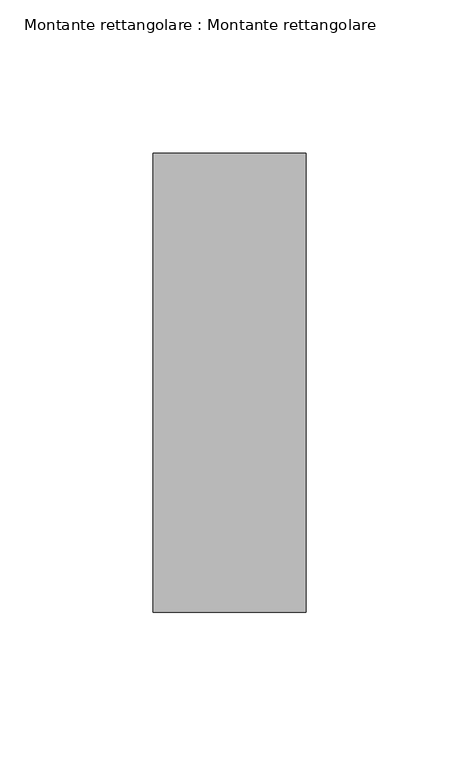
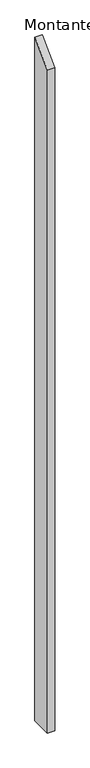
"""IFC4 building model written with IfcOpenShell, lengths in millimetres: member geometry, Montante rettangolare : Montante rettangolare."""

from ifc_helpers import new_model, si_unit, frame, origin, place, context, project, spatial, polyline, outline, extrude, source, transform, mapped, element, save


def montante_rettangolare_montante_rettangolare_f37d3d93(model_context):
    return source(origin(), model_context, "Body", "SweptSolid", [
        extrude(outline(polyline([(-75.0, -75.0), (75.0, 75.0), (75.0, -4920.0), (-75.0, -4920.0), (-75.0, -75.0)])), frame((-50.0, 0.0, 0.0), z_axis=(1.0, 0.0, 0.0), x_axis=(0.0, 1.0, 0.0)), (0.0, 0.0, 1.0), 50.0),
    ])


if __name__ == "__main__":
    model = new_model("IFC4")
    model_context = context("Model", 3, world=origin())
    ifc_project = project(units=[si_unit("LENGTHUNIT", "METRE", prefix="MILLI")], contexts=[model_context])
    site = spatial("IfcSite", under=ifc_project)
    building = spatial("IfcBuilding", under=site)
    placement = place(None, origin())
    montante_rettangolare_montante_rettangolare_shape = montante_rettangolare_montante_rettangolare_f37d3d93(model_context)
    element("IfcMember", 1, ObjectType="Montante rettangolare : Montante rettangolare", at=placement, inside=building, context=model_context, shape_type="MappedRepresentation", body=[
        mapped(montante_rettangolare_montante_rettangolare_shape, transform((0.0, 0.0, 0.0), x_axis=(1.0, 0.0, 0.0), y_axis=(0.0, 1.0, 0.0), z_axis=(0.0, 0.0, 1.0))),
    ])
    save(model, "model.ifc")

# Revit data of these elements
# Type "Montante rettangolare : Montante rettangolare"
#   built-in parameter 1007304 = 0.492126 (stored number, unit not read)
#   built-in parameter 1007301 = 0.082021 (stored number, unit not read)
#   built-in parameter 1007300 = 0.082021 (stored number, unit not read)
# Element 1 (IfcMember, "Montante rettangolare : Montante rettangolare")
#   Materials on its faces: "Acciaio"
# Materials
#   "Acciaio": class "Metallo", colour RGB 247 247 247, transparency 0, Description = "Acciaio, finitura zigrinata", Cost = 0
